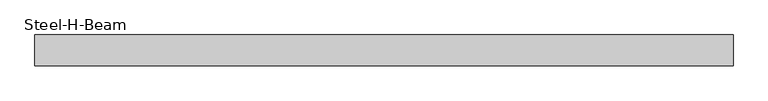
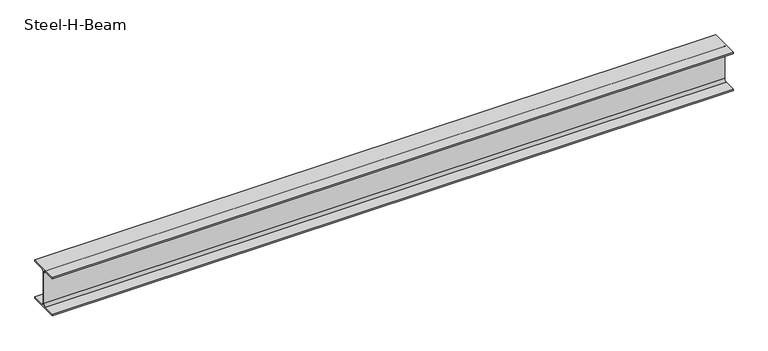
"""IFC4 building model written with IfcOpenShell, lengths in millimetres: beam geometry, Steel-H-Beam : BM121_H-340×250x9x14."""

from ifc_helpers import new_model, si_unit, point, frame, frame_2d, origin, place, context, project, spatial, polyline, circle_curve, trimmed, segment, composite_curve, outline, extrude, source, transform, mapped, element, save


def steel_h_beam_0febaaa8(model_context):
    return source(origin(), model_context, "Body", "SweptSolid", [
        extrude(outline(composite_curve([segment(polyline([(125.0, -156.0), (125.0, -170.0), (-125.0, -170.0), (-125.0, -156.0), (-24.5, -156.0)]), True, "CONTINUOUS"), segment(trimmed(circle_curve(frame_2d((-24.5, -136.0)), 20.0), [point((-24.5, -156.0))], [point((-4.5, -136.0))], True, "CARTESIAN"), True, "CONTINUOUS"), segment(polyline([(-4.5, -136.0), (-4.5, 136.0)]), True, "CONTINUOUS"), segment(trimmed(circle_curve(frame_2d((-24.5, 136.0)), 20.0), [point((-4.5, 136.0))], [point((-24.5, 156.0))], True, "CARTESIAN"), True, "CONTINUOUS"), segment(polyline([(-24.5, 156.0), (-125.0, 156.0), (-125.0, 170.0), (125.0, 170.0), (125.0, 156.0), (24.5, 156.0)]), True, "CONTINUOUS"), segment(trimmed(circle_curve(frame_2d((24.5, 136.0)), 20.0), [point((24.5, 156.0))], [point((4.5, 136.0))], True, "CARTESIAN"), True, "CONTINUOUS"), segment(polyline([(4.5, 136.0), (4.5, -136.0)]), True, "CONTINUOUS"), segment(trimmed(circle_curve(frame_2d((24.5, -136.0)), 20.0), [point((4.5, -136.0))], [point((24.5, -156.0))], True, "CARTESIAN"), True, "CONTINUOUS"), segment(polyline([(24.5, -156.0), (125.0, -156.0)]), True, "CONTINUOUS")], self_intersect=False)), frame((-2854.7871653, 0.0, 0.0), z_axis=(1.0, 0.0, 0.0), x_axis=(0.0, 1.0, 0.0)), (0.0, 0.0, 1.0), 5681.370928),
    ])


if __name__ == "__main__":
    model = new_model("IFC4")
    model_context = context("Model", 3, world=origin())
    ifc_project = project(units=[si_unit("LENGTHUNIT", "METRE", prefix="MILLI")], contexts=[model_context])
    site = spatial("IfcSite", under=ifc_project)
    building = spatial("IfcBuilding", under=site)
    placement = place(None, origin())
    steel_h_beam_shape = steel_h_beam_0febaaa8(model_context)
    element("IfcBeam", 1, ObjectType="Steel-H-Beam : BM121_H-340×250x9x14", at=placement, inside=building, context=model_context, shape_type="MappedRepresentation", body=[
        mapped(steel_h_beam_shape, transform((0.0, 0.0, 0.0), x_axis=(1.0, 0.0, 0.0), y_axis=(0.0, 1.0, 0.0), z_axis=(0.0, 0.0, 1.0))),
    ])
    save(model, "model.ifc")

# Revit data of these elements
# Type "Steel-H-Beam : BM121_H-340×250x9x14"
#   Surface Area = 1.62766 m²/m
#   Section Area = 101.514 cm²
#   Mass per Unit Length = 79.6882 kg/m
#   Length [instance default] = 3000 mm
#   B = 250 mm
#   H = 340 mm
#   r = 20 mm
#   tw = 9 mm
#   tf = 14 mm
#   hec_material4 [instance default] = none
#   hec_material3 [instance default] = none
#   hec_material2 [instance default] = none
#   hec_material1 [instance default] = none
#   Structural Material [instance default] = Steel, 45-345
#   Assembly Code = ""
# Element 1 (IfcBeam, "Steel-H-Beam : BM121_H-340×250x9x14")
#   hec_material4 = S01AA010-00002_Main Steel Structure Fabrication Work_Shelter/Building_Steel Painting/Coating_for Fireproofed Steel Surface, Surface Preparation & Primer Coat
#   hec_material3 = F01AC000-00002_Building/Shelter Fire Proofing Work_Intumescent Coating Type_1 hr. rating (UL 1709))
#   hec_material2 = S01AA010-00002_Main Steel Structure Fabrication Work_Shelter/Building_Steel Painting/Coating_for Fireproofed Steel Surface, Surface Preparation & Primer Coat
#   hec_material1 = S03AA028-00001_Main Steel Structure Erection Work_Shelter/Building_Medium Steel
#   Structural Material = S01AA002-00001_Main Steel Structure Fabrication Work_Shelter/Building_Medium Steel - Standard
#   Materials on its faces: "S01AA002-00001_Main Steel Structure Fabrication Work_Shelter/Building_Medium Steel - Standard"
# Materials
#   "Steel, 45-345": class "Metal", colour RGB 189 187 185, transparency 0, Description = "Steel 345 MPa", Cost = 0
#   "S01AA002-00001_Main Steel Structure Fabrication Work_Shelter/Building_Medium Steel - Standard": class "Metal", colour RGB 120 120 120, transparency 0, Comments = "(90KG/M>Weight≥30KG/M)", Description = "Structural steel 50ksi", W00) Work Master Code = "S01AA002-0001", W01) Work Master_Lv1 = "Main Steel Structure Fabrication Work", W02) Work Master_Lv2 = "Shelter/Building", W03) Work Master_Spec.1 = "Medium Steel - Standard (90KG/M>Weight≥30KG/M)", Cost = 0
#   "S01AA010-00002_Main Steel Structure Fabrication Work_Shelter/Building_Steel Painting/Coating_for Fireproofed Steel Surface, Surface Preparation & Primer Coat": class "Metal", colour RGB 120 120 120, transparency 0, Description = "Paint finished steel", W00) Work Master Code = "SS01AA010-00002", W01) Work Master_Lv1 = "Main Steel Structure Fabrication Work", W02) Work Master_Lv2 = "Shelter/Building", W03) Work Master_Spec.1 = "Steel Painting/Coating", W04) Work Master_Spec.2 = "for Fireproofed Steel Surface, Surface Preparation & Primer Coat", Cost = 0
#   "F01AC000-00002_Building/Shelter Fire Proofing Work_Intumescent Coating Type_1 hr. rating (UL 1709))": class "Metal", colour RGB 255 128 128, transparency 0, Description = "Paint finished steel", W00) Work Master Code = "F01AC000-00002", W01) Work Master_Lv1 = "Building/Shelter Fire Proofing Work", W02) Work Master_Lv2 = "Intumescent Coating Type", W03) Work Master_Spec.1 = "1 hr. rating (UL 1709)", Cost = 0
#   "S03AA028-00001_Main Steel Structure Erection Work_Shelter/Building_Medium Steel": class "Metal", colour RGB 120 120 120, transparency 0, Comments = "(90KG/M>Weight≥30KG/M)", Description = "Structural steel 50ksi", W00) Work Master Code = "S03AA028-0001", W01) Work Master_Lv1 = "Main Steel Structure Erection Work", W02) Work Master_Lv2 = "Shelter/Building", W03) Work Master_Spec.1 = "Medium Steel (90KG/M>Weight≥30KG/M)", Cost = 0
